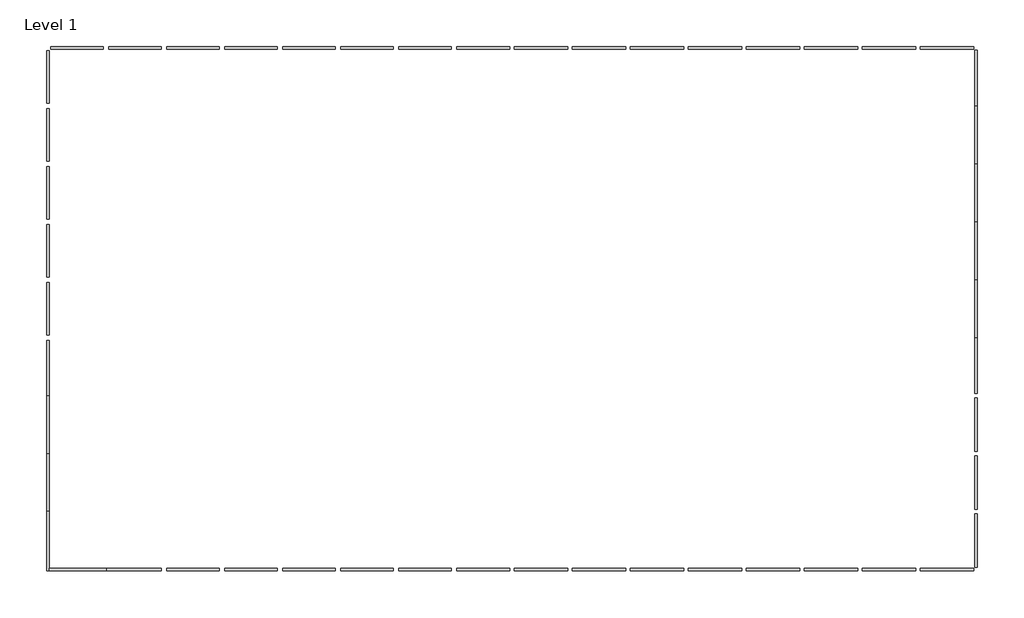
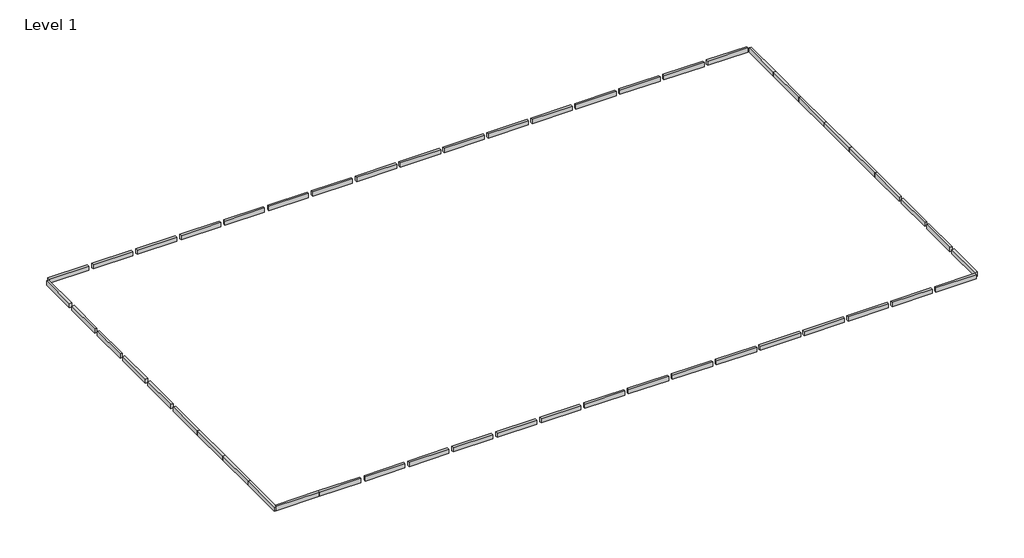
# One storey: 50 beams.
"""IFC4 building model written with IfcOpenShell, lengths in millimetres."""

from ifc_helpers import new_model, si_unit, frame, origin, place, context, project, spatial, polyline, outline, extrude, faceted_brep, element, save

model = new_model("IFC4")

# Units and contexts
model_context = context("Model", 3, world=origin())
ifc_project = project(units=[si_unit("LENGTHUNIT", "METRE", prefix="MILLI")], contexts=[model_context])

# Site, building, storey
site = spatial("IfcSite", under=ifc_project)
building = spatial("IfcBuilding", under=site)
storey = spatial("IfcBuildingStorey", under=building, Name="Level 1", Elevation=0.0)

# Beams
placement = place(None, origin())
element("IfcBeam", 1, ObjectType="BM111_Concrete-Rectangular Beam : BM111_400x600", at=placement, inside=storey, context=model_context, shape_type="SweptSolid", body=[
    extrude(outline(polyline([(96152.4, -6000.0), (95847.6, -6000.0), (95847.6, -250.0), (96152.4, -250.0), (96152.4, -6000.0)])), frame((0.0, 0.0, -609.6), z_axis=(0.0, 0.0, 1.0), x_axis=(1.0, 0.0, 0.0)), (0.0, 0.0, 1.0), 609.6),
])
element("IfcBeam", 2, ObjectType="BM111_Concrete-Rectangular Beam : BM111_400x600", at=placement, inside=storey, context=model_context, shape_type="SweptSolid", body=[
    extrude(outline(polyline([(-152.4, -300.0), (152.4, -300.0), (152.4, -5700.0), (-152.4, -5700.0), (-152.4, -300.0)])), frame((0.0, 0.0, -609.6), z_axis=(0.0, 0.0, 1.0), x_axis=(1.0, 0.0, 0.0)), (0.0, 0.0, 1.0), 609.6),
])
element("IfcBeam", 3, ObjectType="BM111_Concrete-Rectangular Beam : BM111_400x600", at=placement, inside=storey, context=model_context, shape_type="SweptSolid", body=[
    extrude(outline(polyline([(96152.4, -12000.0), (95847.6, -12000.0), (95847.6, -6000.0), (96152.4, -6000.0), (96152.4, -12000.0)])), frame((0.0, 0.0, -609.6), z_axis=(0.0, 0.0, 1.0), x_axis=(1.0, 0.0, 0.0)), (0.0, 0.0, 1.0), 609.6),
])
element("IfcBeam", 4, ObjectType="BM111_Concrete-Rectangular Beam : BM111_400x600", at=placement, inside=storey, context=model_context, shape_type="SweptSolid", body=[
    extrude(outline(polyline([(152.4, -11700.0), (-152.4, -11700.0), (-152.4, -6300.0), (152.4, -6300.0), (152.4, -11700.0)])), frame((0.0, 0.0, -609.6), z_axis=(0.0, 0.0, 1.0), x_axis=(1.0, 0.0, 0.0)), (0.0, 0.0, 1.0), 609.6),
])
element("IfcBeam", 5, ObjectType="BM111_Concrete-Rectangular Beam : BM111_400x600", at=placement, inside=storey, context=model_context, shape_type="SweptSolid", body=[
    extrude(outline(polyline([(96152.4, -18000.0), (95847.6, -18000.0), (95847.6, -12000.0), (96152.4, -12000.0), (96152.4, -18000.0)])), frame((0.0, 0.0, -609.6), z_axis=(0.0, 0.0, 1.0), x_axis=(1.0, 0.0, 0.0)), (0.0, 0.0, 1.0), 609.6),
])
element("IfcBeam", 6, ObjectType="BM111_Concrete-Rectangular Beam : BM111_400x600", at=placement, inside=storey, context=model_context, shape_type="SweptSolid", body=[
    extrude(outline(polyline([(152.4, -17700.0), (-152.4, -17700.0), (-152.4, -12300.0), (152.4, -12300.0), (152.4, -17700.0)])), frame((0.0, 0.0, -609.6), z_axis=(0.0, 0.0, 1.0), x_axis=(1.0, 0.0, 0.0)), (0.0, 0.0, 1.0), 609.6),
])
element("IfcBeam", 7, ObjectType="BM111_Concrete-Rectangular Beam : BM111_400x600", at=placement, inside=storey, context=model_context, shape_type="SweptSolid", body=[
    extrude(outline(polyline([(96152.4, -24000.0), (95847.6, -24000.0), (95847.6, -18000.0), (96152.4, -18000.0), (96152.4, -24000.0)])), frame((0.0, 0.0, -609.6), z_axis=(0.0, 0.0, 1.0), x_axis=(1.0, 0.0, 0.0)), (0.0, 0.0, 1.0), 609.6),
])
element("IfcBeam", 8, ObjectType="BM111_Concrete-Rectangular Beam : BM111_400x600", at=placement, inside=storey, context=model_context, shape_type="SweptSolid", body=[
    extrude(outline(polyline([(152.4, -23700.0), (-152.4, -23700.0), (-152.4, -18300.0), (152.4, -18300.0), (152.4, -23700.0)])), frame((0.0, 0.0, -609.6), z_axis=(0.0, 0.0, 1.0), x_axis=(1.0, 0.0, 0.0)), (0.0, 0.0, 1.0), 609.6),
])
element("IfcBeam", 9, ObjectType="BM111_Concrete-Rectangular Beam : BM111_400x600", at=placement, inside=storey, context=model_context, shape_type="SweptSolid", body=[
    extrude(outline(polyline([(96152.4, -30000.0), (95847.6, -30000.0), (95847.6, -24000.0), (96152.4, -24000.0), (96152.4, -30000.0)])), frame((0.0, 0.0, -609.6), z_axis=(0.0, 0.0, 1.0), x_axis=(1.0, 0.0, 0.0)), (0.0, 0.0, 1.0), 609.6),
])
element("IfcBeam", 10, ObjectType="BM111_Concrete-Rectangular Beam : BM111_400x600", at=placement, inside=storey, context=model_context, shape_type="SweptSolid", body=[
    extrude(outline(polyline([(-152.4, -24300.0), (152.4, -24300.0), (152.4, -29700.0), (-152.4, -29700.0), (-152.4, -24300.0)])), frame((0.0, 0.0, -609.6), z_axis=(0.0, 0.0, 1.0), x_axis=(1.0, 0.0, 0.0)), (0.0, 0.0, 1.0), 609.6),
])
element("IfcBeam", 11, ObjectType="BM111_Concrete-Rectangular Beam : BM111_400x600", at=placement, inside=storey, context=model_context, shape_type="SweptSolid", body=[
    extrude(outline(polyline([(95847.6, -30000.0), (96152.4, -30000.0), (96152.4, -35750.0), (95847.6, -35750.0), (95847.6, -30000.0)])), frame((0.0, 0.0, -609.6), z_axis=(0.0, 0.0, 1.0), x_axis=(1.0, 0.0, 0.0)), (0.0, 0.0, 1.0), 609.6),
])
element("IfcBeam", 12, ObjectType="BM111_Concrete-Rectangular Beam : BM111_400x600", at=placement, inside=storey, context=model_context, shape_type="SweptSolid", body=[
    extrude(outline(polyline([(152.4, -36000.0), (-152.4, -36000.0), (-152.4, -30300.0), (152.4, -30300.0), (152.4, -36000.0)])), frame((0.0, 0.0, -609.6), z_axis=(0.0, 0.0, 1.0), x_axis=(1.0, 0.0, 0.0)), (0.0, 0.0, 1.0), 609.6),
])
element("IfcBeam", 13, ObjectType="BM111_Concrete-Rectangular Beam : BM111_400x600", at=placement, inside=storey, context=model_context, shape_type="SweptSolid", body=[
    extrude(outline(polyline([(95847.6, -36250.0), (96152.4, -36250.0), (96152.4, -41750.0), (95847.6, -41750.0), (95847.6, -36250.0)])), frame((0.0, 0.0, -609.6), z_axis=(0.0, 0.0, 1.0), x_axis=(1.0, 0.0, 0.0)), (0.0, 0.0, 1.0), 609.6),
])
element("IfcBeam", 14, ObjectType="BM111_Concrete-Rectangular Beam : BM111_400x600", at=placement, inside=storey, context=model_context, shape_type="SweptSolid", body=[
    extrude(outline(polyline([(152.4, -42000.0), (-152.4, -42000.0), (-152.4, -36000.0), (152.4, -36000.0), (152.4, -42000.0)])), frame((0.0, 0.0, -609.6), z_axis=(0.0, 0.0, 1.0), x_axis=(1.0, 0.0, 0.0)), (0.0, 0.0, 1.0), 609.6),
])
element("IfcBeam", 15, ObjectType="BM111_Concrete-Rectangular Beam : BM111_400x600", at=placement, inside=storey, context=model_context, shape_type="SweptSolid", body=[
    extrude(outline(polyline([(96152.4, -47750.0), (95847.6, -47750.0), (95847.6, -42250.0), (96152.4, -42250.0), (96152.4, -47750.0)])), frame((0.0, 0.0, -609.6), z_axis=(0.0, 0.0, 1.0), x_axis=(1.0, 0.0, 0.0)), (0.0, 0.0, 1.0), 609.6),
])
element("IfcBeam", 16, ObjectType="BM111_Concrete-Rectangular Beam : BM111_400x600", at=placement, inside=storey, context=model_context, shape_type="SweptSolid", body=[
    extrude(outline(polyline([(152.4, -48000.0), (-152.4, -48000.0), (-152.4, -42000.0), (152.4, -42000.0), (152.4, -48000.0)])), frame((0.0, 0.0, -609.6), z_axis=(0.0, 0.0, 1.0), x_axis=(1.0, 0.0, 0.0)), (0.0, 0.0, 1.0), 609.6),
])
element("IfcBeam", 17, ObjectType="BM111_Concrete-Rectangular Beam : BM111_400x600", at=placement, inside=storey, context=model_context, shape_type="SweptSolid", body=[
    extrude(outline(polyline([(95847.6, -48250.0), (96152.4, -48250.0), (96152.4, -53750.0), (95847.6, -53750.0), (95847.6, -48250.0)])), frame((0.0, 0.0, -609.6), z_axis=(0.0, 0.0, 1.0), x_axis=(1.0, 0.0, 0.0)), (0.0, 0.0, 1.0), 609.6),
])
element("IfcBeam", 18, ObjectType="BM111_Concrete-Rectangular Beam : BM111_400x600", at=placement, inside=storey, context=model_context, shape_type="Brep", body=[
    faceted_brep([(152.4, -48000.0, 0.0), (-152.4, -48000.0, 0.0), (-152.4, -54152.4, 0.0), (152.4, -54152.4, 0.0), (152.4, -53847.6, 0.0), (-152.4, -48000.0, -609.6), (-152.4, -54152.4, -609.6), (152.4, -48000.0, -609.6), (152.4, -53847.6, -609.6), (152.4, -54152.4, -609.6)], [[[0, 1, 2, 3, 4]], [[1, 5, 6, 2]], [[5, 7, 8, 9, 6]], [[7, 0, 4, 3, 9, 8]], [[3, 2, 6, 9]], [[0, 7, 5, 1]]]),
])
element("IfcBeam", 19, ObjectType="BM111_Concrete-Rectangular Beam : BM111_400x600", at=placement, inside=storey, context=model_context, shape_type="SweptSolid", body=[
    extrude(outline(polyline([(18300.0, -152.4), (18300.0, 152.4), (23700.0, 152.4), (23700.0, -152.4), (18300.0, -152.4)])), frame((0.0, 0.0, -609.6), z_axis=(0.0, 0.0, 1.0), x_axis=(1.0, 0.0, 0.0)), (0.0, 0.0, 1.0), 609.6),
])
element("IfcBeam", 20, ObjectType="BM111_Concrete-Rectangular Beam : BM111_400x600", at=placement, inside=storey, context=model_context, shape_type="SweptSolid", body=[
    extrude(outline(polyline([(24300.0, -152.4), (24300.0, 152.4), (29700.0, 152.4), (29700.0, -152.4), (24300.0, -152.4)])), frame((0.0, 0.0, -609.6), z_axis=(0.0, 0.0, 1.0), x_axis=(1.0, 0.0, 0.0)), (0.0, 0.0, 1.0), 609.6),
])
element("IfcBeam", 21, ObjectType="BM111_Concrete-Rectangular Beam : BM111_400x600", at=placement, inside=storey, context=model_context, shape_type="SweptSolid", body=[
    extrude(outline(polyline([(30300.0, -152.4), (30300.0, 152.4), (35700.0, 152.4), (35700.0, -152.4), (30300.0, -152.4)])), frame((0.0, 0.0, -609.6), z_axis=(0.0, 0.0, 1.0), x_axis=(1.0, 0.0, 0.0)), (0.0, 0.0, 1.0), 609.6),
])
element("IfcBeam", 22, ObjectType="BM111_Concrete-Rectangular Beam : BM111_400x600", at=placement, inside=storey, context=model_context, shape_type="SweptSolid", body=[
    extrude(outline(polyline([(36300.0, -152.4), (36300.0, 152.4), (41700.0, 152.4), (41700.0, -152.4), (36300.0, -152.4)])), frame((0.0, 0.0, -609.6), z_axis=(0.0, 0.0, 1.0), x_axis=(1.0, 0.0, 0.0)), (0.0, 0.0, 1.0), 609.6),
])
element("IfcBeam", 23, ObjectType="BM111_Concrete-Rectangular Beam : BM111_400x600", at=placement, inside=storey, context=model_context, shape_type="SweptSolid", body=[
    extrude(outline(polyline([(300.0, -152.4), (300.0, 152.4), (5700.0, 152.4), (5700.0, -152.4), (300.0, -152.4)])), frame((0.0, 0.0, -609.6), z_axis=(0.0, 0.0, 1.0), x_axis=(1.0, 0.0, 0.0)), (0.0, 0.0, 1.0), 609.6),
])
element("IfcBeam", 24, ObjectType="BM111_Concrete-Rectangular Beam : BM111_400x600", at=placement, inside=storey, context=model_context, shape_type="SweptSolid", body=[
    extrude(outline(polyline([(6300.0, -152.4), (6300.0, 152.4), (11700.0, 152.4), (11700.0, -152.4), (6300.0, -152.4)])), frame((0.0, 0.0, -609.6), z_axis=(0.0, 0.0, 1.0), x_axis=(1.0, 0.0, 0.0)), (0.0, 0.0, 1.0), 609.6),
])
element("IfcBeam", 25, ObjectType="BM111_Concrete-Rectangular Beam : BM111_400x600", at=placement, inside=storey, context=model_context, shape_type="SweptSolid", body=[
    extrude(outline(polyline([(17700.0, 152.4), (17700.0, -152.4), (12300.0, -152.4), (12300.0, 152.4), (17700.0, 152.4)])), frame((0.0, 0.0, -609.6), z_axis=(0.0, 0.0, 1.0), x_axis=(1.0, 0.0, 0.0)), (0.0, 0.0, 1.0), 609.6),
])
element("IfcBeam", 26, ObjectType="BM111_Concrete-Rectangular Beam : BM111_400x600", at=placement, inside=storey, context=model_context, shape_type="SweptSolid", body=[
    extrude(outline(polyline([(42300.0, -152.4), (42300.0, 152.4), (47750.0, 152.4), (47750.0, -152.4), (42300.0, -152.4)])), frame((0.0, 0.0, -609.6), z_axis=(0.0, 0.0, 1.0), x_axis=(1.0, 0.0, 0.0)), (0.0, 0.0, 1.0), 609.6),
])
element("IfcBeam", 27, ObjectType="BM111_Concrete-Rectangular Beam : BM111_400x600", at=placement, inside=storey, context=model_context, shape_type="SweptSolid", body=[
    extrude(outline(polyline([(53750.0, 152.4), (53750.0, -152.4), (48250.0, -152.4), (48250.0, 152.4), (53750.0, 152.4)])), frame((0.0, 0.0, -609.6), z_axis=(0.0, 0.0, 1.0), x_axis=(1.0, 0.0, 0.0)), (0.0, 0.0, 1.0), 609.6),
])
element("IfcBeam", 28, ObjectType="BM111_Concrete-Rectangular Beam : BM111_400x600", at=placement, inside=storey, context=model_context, shape_type="SweptSolid", body=[
    extrude(outline(polyline([(83750.0, 152.4), (83750.0, -152.4), (78250.0, -152.4), (78250.0, 152.4), (83750.0, 152.4)])), frame((0.0, 0.0, -609.6), z_axis=(0.0, 0.0, 1.0), x_axis=(1.0, 0.0, 0.0)), (0.0, 0.0, 1.0), 609.6),
])
element("IfcBeam", 29, ObjectType="BM111_Concrete-Rectangular Beam : BM111_400x600", at=placement, inside=storey, context=model_context, shape_type="SweptSolid", body=[
    extrude(outline(polyline([(84250.0, -152.4), (84250.0, 152.4), (89750.0, 152.4), (89750.0, -152.4), (84250.0, -152.4)])), frame((0.0, 0.0, -609.6), z_axis=(0.0, 0.0, 1.0), x_axis=(1.0, 0.0, 0.0)), (0.0, 0.0, 1.0), 609.6),
])
element("IfcBeam", 30, ObjectType="BM111_Concrete-Rectangular Beam : BM111_400x600", at=placement, inside=storey, context=model_context, shape_type="SweptSolid", body=[
    extrude(outline(polyline([(90250.0, -152.4), (90250.0, 152.4), (95750.0, 152.4), (95750.0, -152.4), (90250.0, -152.4)])), frame((0.0, 0.0, -609.6), z_axis=(0.0, 0.0, 1.0), x_axis=(1.0, 0.0, 0.0)), (0.0, 0.0, 1.0), 609.6),
])
element("IfcBeam", 31, ObjectType="BM111_Concrete-Rectangular Beam : BM111_400x600", at=placement, inside=storey, context=model_context, shape_type="SweptSolid", body=[
    extrude(outline(polyline([(54250.0, -152.4), (54250.0, 152.4), (59750.0, 152.4), (59750.0, -152.4), (54250.0, -152.4)])), frame((0.0, 0.0, -609.6), z_axis=(0.0, 0.0, 1.0), x_axis=(1.0, 0.0, 0.0)), (0.0, 0.0, 1.0), 609.6),
])
element("IfcBeam", 32, ObjectType="BM111_Concrete-Rectangular Beam : BM111_400x600", at=placement, inside=storey, context=model_context, shape_type="SweptSolid", body=[
    extrude(outline(polyline([(60250.0, -152.4), (60250.0, 152.4), (65750.0, 152.4), (65750.0, -152.4), (60250.0, -152.4)])), frame((0.0, 0.0, -609.6), z_axis=(0.0, 0.0, 1.0), x_axis=(1.0, 0.0, 0.0)), (0.0, 0.0, 1.0), 609.6),
])
element("IfcBeam", 33, ObjectType="BM111_Concrete-Rectangular Beam : BM111_400x600", at=placement, inside=storey, context=model_context, shape_type="SweptSolid", body=[
    extrude(outline(polyline([(71750.0, 152.4), (71750.0, -152.4), (66250.0, -152.4), (66250.0, 152.4), (71750.0, 152.4)])), frame((0.0, 0.0, -609.6), z_axis=(0.0, 0.0, 1.0), x_axis=(1.0, 0.0, 0.0)), (0.0, 0.0, 1.0), 609.6),
])
element("IfcBeam", 34, ObjectType="BM111_Concrete-Rectangular Beam : BM111_400x600", at=placement, inside=storey, context=model_context, shape_type="SweptSolid", body=[
    extrude(outline(polyline([(72250.0, -152.4), (72250.0, 152.4), (77750.0, 152.4), (77750.0, -152.4), (72250.0, -152.4)])), frame((0.0, 0.0, -609.6), z_axis=(0.0, 0.0, 1.0), x_axis=(1.0, 0.0, 0.0)), (0.0, 0.0, 1.0), 609.6),
])
element("IfcBeam", 35, ObjectType="BM111_Concrete-Rectangular Beam : BM111_400x600", at=placement, inside=storey, context=model_context, shape_type="SweptSolid", body=[
    extrude(outline(polyline([(23700.0, -53847.6), (23700.0, -54152.4), (18300.0, -54152.4), (18300.0, -53847.6), (23700.0, -53847.6)])), frame((0.0, 0.0, -609.6), z_axis=(0.0, 0.0, 1.0), x_axis=(1.0, 0.0, 0.0)), (0.0, 0.0, 1.0), 609.6),
])
element("IfcBeam", 36, ObjectType="BM111_Concrete-Rectangular Beam : BM111_400x600", at=placement, inside=storey, context=model_context, shape_type="SweptSolid", body=[
    extrude(outline(polyline([(29700.0, -53847.6), (29700.0, -54152.4), (24300.0, -54152.4), (24300.0, -53847.6), (29700.0, -53847.6)])), frame((0.0, 0.0, -609.6), z_axis=(0.0, 0.0, 1.0), x_axis=(1.0, 0.0, 0.0)), (0.0, 0.0, 1.0), 609.6),
])
element("IfcBeam", 37, ObjectType="BM111_Concrete-Rectangular Beam : BM111_400x600", at=placement, inside=storey, context=model_context, shape_type="SweptSolid", body=[
    extrude(outline(polyline([(35700.0, -53847.6), (35700.0, -54152.4), (30300.0, -54152.4), (30300.0, -53847.6), (35700.0, -53847.6)])), frame((0.0, 0.0, -609.6), z_axis=(0.0, 0.0, 1.0), x_axis=(1.0, 0.0, 0.0)), (0.0, 0.0, 1.0), 609.6),
])
element("IfcBeam", 38, ObjectType="BM111_Concrete-Rectangular Beam : BM111_400x600", at=placement, inside=storey, context=model_context, shape_type="SweptSolid", body=[
    extrude(outline(polyline([(41700.0, -53847.6), (41700.0, -54152.4), (36300.0, -54152.4), (36300.0, -53847.6), (41700.0, -53847.6)])), frame((0.0, 0.0, -609.6), z_axis=(0.0, 0.0, 1.0), x_axis=(1.0, 0.0, 0.0)), (0.0, 0.0, 1.0), 609.6),
])
element("IfcBeam", 39, ObjectType="BM111_Concrete-Rectangular Beam : BM111_400x600", at=placement, inside=storey, context=model_context, shape_type="SweptSolid", body=[
    extrude(outline(polyline([(6000.0, -53847.6), (6000.0, -54152.4), (152.4, -54152.4), (152.4, -53847.6), (6000.0, -53847.6)])), frame((0.0, 0.0, -609.6), z_axis=(0.0, 0.0, 1.0), x_axis=(1.0, 0.0, 0.0)), (0.0, 0.0, 1.0), 609.6),
])
element("IfcBeam", 40, ObjectType="BM111_Concrete-Rectangular Beam : BM111_400x600", at=placement, inside=storey, context=model_context, shape_type="SweptSolid", body=[
    extrude(outline(polyline([(6000.0, -54152.4), (6000.0, -53847.6), (11700.0, -53847.6), (11700.0, -54152.4), (6000.0, -54152.4)])), frame((0.0, 0.0, -609.6), z_axis=(0.0, 0.0, 1.0), x_axis=(1.0, 0.0, 0.0)), (0.0, 0.0, 1.0), 609.6),
])
element("IfcBeam", 41, ObjectType="BM111_Concrete-Rectangular Beam : BM111_400x600", at=placement, inside=storey, context=model_context, shape_type="SweptSolid", body=[
    extrude(outline(polyline([(17700.0, -53847.6), (17700.0, -54152.4), (12300.0, -54152.4), (12300.0, -53847.6), (17700.0, -53847.6)])), frame((0.0, 0.0, -609.6), z_axis=(0.0, 0.0, 1.0), x_axis=(1.0, 0.0, 0.0)), (0.0, 0.0, 1.0), 609.6),
])
element("IfcBeam", 42, ObjectType="BM111_Concrete-Rectangular Beam : BM111_400x600", at=placement, inside=storey, context=model_context, shape_type="SweptSolid", body=[
    extrude(outline(polyline([(47750.0, -53847.6), (47750.0, -54152.4), (42300.0, -54152.4), (42300.0, -53847.6), (47750.0, -53847.6)])), frame((0.0, 0.0, -609.6), z_axis=(0.0, 0.0, 1.0), x_axis=(1.0, 0.0, 0.0)), (0.0, 0.0, 1.0), 609.6),
])
element("IfcBeam", 43, ObjectType="BM111_Concrete-Rectangular Beam : BM111_400x600", at=placement, inside=storey, context=model_context, shape_type="SweptSolid", body=[
    extrude(outline(polyline([(53750.0, -53847.6), (53750.0, -54152.4), (48250.0, -54152.4), (48250.0, -53847.6), (53750.0, -53847.6)])), frame((0.0, 0.0, -609.6), z_axis=(0.0, 0.0, 1.0), x_axis=(1.0, 0.0, 0.0)), (0.0, 0.0, 1.0), 609.6),
])
element("IfcBeam", 44, ObjectType="BM111_Concrete-Rectangular Beam : BM111_400x600", at=placement, inside=storey, context=model_context, shape_type="SweptSolid", body=[
    extrude(outline(polyline([(83750.0, -53847.6), (83750.0, -54152.4), (78250.0, -54152.4), (78250.0, -53847.6), (83750.0, -53847.6)])), frame((0.0, 0.0, -609.6), z_axis=(0.0, 0.0, 1.0), x_axis=(1.0, 0.0, 0.0)), (0.0, 0.0, 1.0), 609.6),
])
element("IfcBeam", 45, ObjectType="BM111_Concrete-Rectangular Beam : BM111_400x600", at=placement, inside=storey, context=model_context, shape_type="SweptSolid", body=[
    extrude(outline(polyline([(84250.0, -54152.4), (84250.0, -53847.6), (89750.0, -53847.6), (89750.0, -54152.4), (84250.0, -54152.4)])), frame((0.0, 0.0, -609.6), z_axis=(0.0, 0.0, 1.0), x_axis=(1.0, 0.0, 0.0)), (0.0, 0.0, 1.0), 609.6),
])
element("IfcBeam", 46, ObjectType="BM111_Concrete-Rectangular Beam : BM111_400x600", at=placement, inside=storey, context=model_context, shape_type="SweptSolid", body=[
    extrude(outline(polyline([(90250.0, -54152.4), (90250.0, -53847.6), (95750.0, -53847.6), (95750.0, -54152.4), (90250.0, -54152.4)])), frame((0.0, 0.0, -609.6), z_axis=(0.0, 0.0, 1.0), x_axis=(1.0, 0.0, 0.0)), (0.0, 0.0, 1.0), 609.6),
])
element("IfcBeam", 47, ObjectType="BM111_Concrete-Rectangular Beam : BM111_400x600", at=placement, inside=storey, context=model_context, shape_type="SweptSolid", body=[
    extrude(outline(polyline([(54250.0, -54152.4), (54250.0, -53847.6), (59750.0, -53847.6), (59750.0, -54152.4), (54250.0, -54152.4)])), frame((0.0, 0.0, -609.6), z_axis=(0.0, 0.0, 1.0), x_axis=(1.0, 0.0, 0.0)), (0.0, 0.0, 1.0), 609.6),
])
element("IfcBeam", 48, ObjectType="BM111_Concrete-Rectangular Beam : BM111_400x600", at=placement, inside=storey, context=model_context, shape_type="SweptSolid", body=[
    extrude(outline(polyline([(60250.0, -54152.4), (60250.0, -53847.6), (65750.0, -53847.6), (65750.0, -54152.4), (60250.0, -54152.4)])), frame((0.0, 0.0, -609.6), z_axis=(0.0, 0.0, 1.0), x_axis=(1.0, 0.0, 0.0)), (0.0, 0.0, 1.0), 609.6),
])
element("IfcBeam", 49, ObjectType="BM111_Concrete-Rectangular Beam : BM111_400x600", at=placement, inside=storey, context=model_context, shape_type="SweptSolid", body=[
    extrude(outline(polyline([(71750.0, -53847.6), (71750.0, -54152.4), (66250.0, -54152.4), (66250.0, -53847.6), (71750.0, -53847.6)])), frame((0.0, 0.0, -609.6), z_axis=(0.0, 0.0, 1.0), x_axis=(1.0, 0.0, 0.0)), (0.0, 0.0, 1.0), 609.6),
])
element("IfcBeam", 50, ObjectType="BM111_Concrete-Rectangular Beam : BM111_400x600", at=placement, inside=storey, context=model_context, shape_type="SweptSolid", body=[
    extrude(outline(polyline([(72250.0, -54152.4), (72250.0, -53847.6), (77750.0, -53847.6), (77750.0, -54152.4), (72250.0, -54152.4)])), frame((0.0, 0.0, -609.6), z_axis=(0.0, 0.0, 1.0), x_axis=(1.0, 0.0, 0.0)), (0.0, 0.0, 1.0), 609.6),
])

save(model, "model.ifc")

# Revit data of these elements
# Type "BM111_Concrete-Rectangular Beam : BM111_400x600"
#   Assembly Code = "B10"
#   Length [instance default] = 1524 mm
#   b = 304.8 mm
#   h = 609.6 mm
#   Structural Material [instance default] = Concrete, Cast-in-Place gray
# Elements 1, 2, 3, 4, 5, 6, 7, 8, 9, 10, 11, 12, 13, 14, 15, 16, 17, 18, 19, 20, 21, 22, 23, 24, 25, 26, 27, 28, 29, 30, 31, 32, 33, 34, 35, 36, 37, 38, 39, 40, 41, 42, 43, 44, 45, 46, 47, 48, 49, 50 (IfcBeam, "BM111_Concrete-Rectangular Beam : BM111_400x600")
#   Structural Material = Concrete, Cast-in-Place gray
#   Phase Created = New Construction
#   Materials on its faces: "Concrete, Cast-in-Place gray"
# Materials
#   "Concrete, Cast-in-Place gray": class "Concrete", colour RGB 192 192 192, transparency 0, Description = "Cast-in-place concrete", Cost = 0
